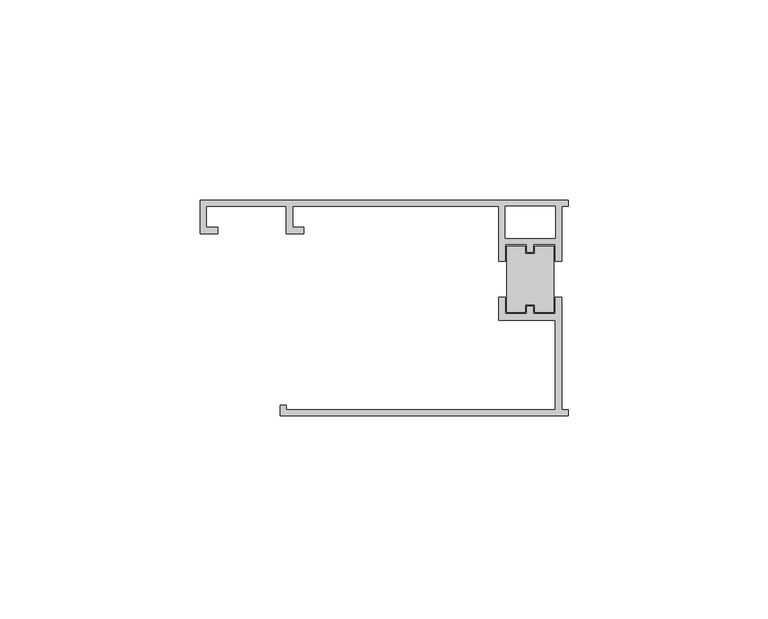
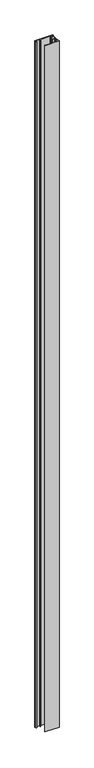
"""IFC4 building model written with IfcOpenShell, lengths in millimetres: proxy geometry, Generic Models 2:Generic Models 2:310765:Generic Models 2:310765 : Generic Models 2:Generic Models 2:310765:6 : Generic Models 2:Generic Models 2:310765:Generic Models 2:310765 : Generic Models 2:Generic Models 2:310765:300385."""

from ifc_helpers import new_model, si_unit, frame, origin, place, context, project, spatial, polyline, outline, extrude, source, transform, mapped, element, save


def generic_models_24953a4c(model_context):
    return source(origin(), model_context, "Body", "SweptSolid", [
        extrude(outline(polyline([(592740.0761017, -579060.466762), (592740.0761017, -579043.9145058), (592744.7736003, -579043.9145058), (592744.7736003, -579045.8399212), (592747.1548503, -579045.8399212), (592747.1548503, -579043.9145058), (592751.8523489, -579043.9145058), (592751.8523489, -579060.466762), (592747.1548503, -579060.466762), (592747.1548503, -579058.5413465), (592744.7736003, -579058.5413465), (592744.7736003, -579060.466762), (592740.0761017, -579060.466762)])), frame((0.0, 0.0, 6.2703961), z_axis=(0.0, 0.0, 1.0), x_axis=(1.0, 0.0, 0.0)), (0.0, 0.0, 1.0), 3695.7),
        extrude(outline(polyline([(592663.4242239, -579040.8458673), (592663.4242239, -579032.3994958), (592755.4242239, -579032.3994958), (592755.4242239, -579033.9869958), (592753.8367239, -579033.9869958), (592753.8367239, -579047.6848183), (592752.2492239, -579047.6848183), (592752.2492239, -579043.5176308), (592746.7579753, -579043.5176308), (592746.7579753, -579045.4430462), (592745.1704753, -579045.4430462), (592745.1704753, -579043.5176308), (592739.6792267, -579043.5176308), (592739.6792267, -579047.6848183), (592738.0917267, -579047.6848183), (592738.0917267, -579033.9869958), (592686.5992239, -579033.9869958), (592686.5992239, -579039.2583673), (592689.3990505, -579039.2583673), (592689.3990505, -579040.8458673), (592685.0117239, -579040.8458673), (592685.0117239, -579033.9869958), (592665.0117239, -579033.9869958), (592665.0117239, -579039.2583673), (592667.8115505, -579039.2583673), (592667.8115505, -579040.8458673), (592663.4242239, -579040.8458673)]), holes=[polyline([(592739.6792267, -579033.9869958), (592739.6792267, -579041.9301308), (592752.2492239, -579041.9301308), (592752.2492239, -579033.9869958), (592739.6792267, -579033.9869958)])]), frame((0.0, 0.0, 6.2703961), z_axis=(0.0, 0.0, 1.0), x_axis=(1.0, 0.0, 0.0)), (0.0, 0.0, 1.0), 3695.7),
        extrude(outline(polyline([(592755.4242239, -579084.8119958), (592755.4242239, -579086.3994958), (592683.4242239, -579086.3994958), (592683.4242239, -579083.6844059), (592685.0117239, -579083.6844059), (592685.0117239, -579084.8119958), (592752.2492239, -579084.8119958), (592752.2492239, -579062.451137), (592738.0917267, -579062.451137), (592738.0917267, -579056.6964495), (592739.6792267, -579056.6964495), (592739.6792267, -579060.863637), (592745.1704753, -579060.863637), (592745.1704753, -579058.9382215), (592746.7579753, -579058.9382215), (592746.7579753, -579060.863637), (592752.2492239, -579060.863637), (592752.2492239, -579056.6964495), (592753.8367239, -579056.6964495), (592753.8367239, -579084.8119958), (592755.4242239, -579084.8119958)])), frame((0.0, 0.0, 6.2703961), z_axis=(0.0, 0.0, 1.0), x_axis=(1.0, 0.0, 0.0)), (0.0, 0.0, 1.0), 3695.7),
    ])


if __name__ == "__main__":
    model = new_model("IFC4")
    model_context = context("Model", 3, world=origin())
    ifc_project = project(units=[si_unit("LENGTHUNIT", "METRE", prefix="MILLI")], contexts=[model_context])
    site = spatial("IfcSite", under=ifc_project)
    building = spatial("IfcBuilding", under=site)
    placement = place(None, origin())
    generic_models_shape = generic_models_24953a4c(model_context)
    element("IfcBuildingElementProxy", 1, Name="Generic Models 2:Generic Models 2:310765:Generic Models 2:310765 : Generic Models 2:Generic Models 2:310765:6 : Generic Models 2:Generic Models 2:310765:Generic Models 2:310765 : Generic Models 2:Generic Models 2:310765:300385", ObjectType="Generic Models 2:Generic Models 2:310765:Generic Models 2:310765 : Generic Models 2:Generic Models 2:310765:6 : Generic Models 2:Generic Models 2:310765:Generic Models 2:310765 : Generic Models 2:Generic Models 2:310765:300385", at=placement, inside=building, context=model_context, shape_type="MappedRepresentation", body=[
        mapped(generic_models_shape, transform((0.0, 0.0, 0.0), x_axis=(1.0, 0.0, 0.0), y_axis=(0.0, 1.0, 0.0), z_axis=(0.0, 0.0, 1.0))),
    ])
    save(model, "model.ifc")

# Revit data of these elements
# Type "Generic Models 2:Generic Models 2:310765:Generic Models 2:310765 : Generic Models 2:Generic Models 2:310765:6 : Generic Models 2:Generic Models 2:310765:Generic Models 2:310765 : Generic Models 2:Generic Models 2:310765:300385"
#   NameOverride = "Generic Models 2:Generic Models 2:310765:Generic Models 2:310765 : Generic Models 2:Generic Models 2:310765:300385"
#   ObjectTypeOverride = "Generic Models 2:310765 : Generic Models 2:Generic Models 2:310765"
#   Reference = "Generic Models 2"
#   Tag = "300385"
# Element 1 (IfcBuildingElementProxy, "Generic Models 2:Generic Models 2:310765:Generic Models 2:310765 : Generic Models 2:Generic Models 2:310765:6 : Generic Models 2:Generic Models 2:310765:Generic Models 2:310765 : Generic Models 2:Generic Models 2:310765:300385")
#   Materials on its faces: "THERMAL BROKEN ALUMINUM STOREFRONT FOR POLYCARBONATE"
# Materials
#   "THERMAL BROKEN ALUMINUM STOREFRONT FOR POLYCARBONATE": class "Unassigned", colour RGB 244 244 244, transparency 0, Keynote = "M07611300.01", Cost = 0
